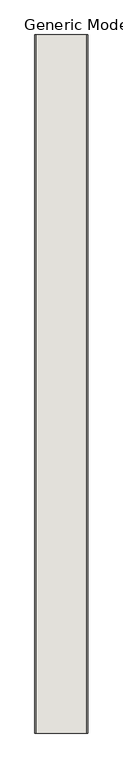
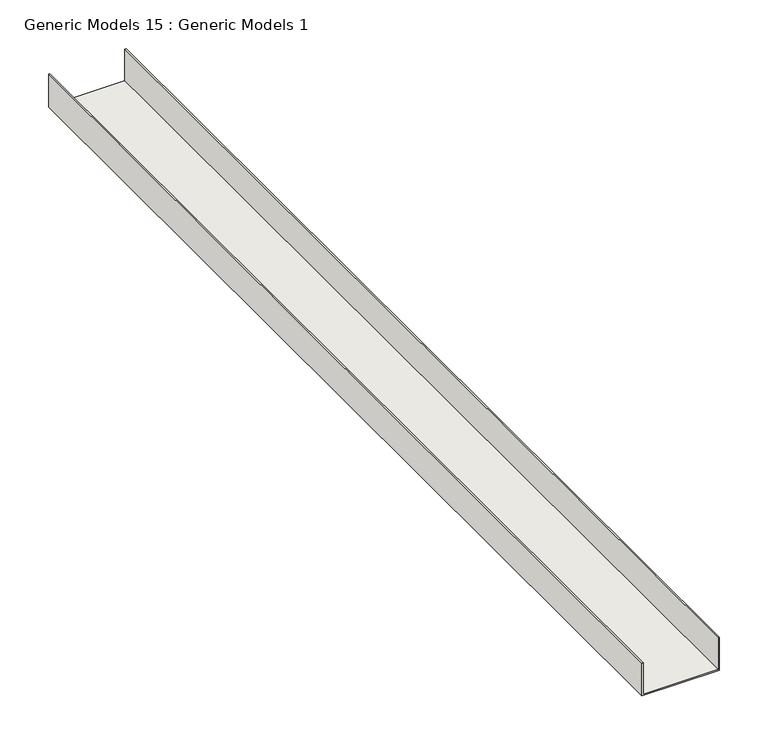
"""IFC4 building model written with IfcOpenShell, lengths in millimetres: wall geometry, Generic Models 15 : Generic Models 1."""

from ifc_helpers import new_model, si_unit, frame, origin, place, context, project, spatial, polyline, outline, extrude, source, transform, mapped, element, save


def generic_models_15_generic_models_1_38d4618c(model_context):
    return source(origin(), model_context, "Body", "SweptSolid", [
        extrude(outline(polyline([(0.0, 49784.0), (41.275, 49784.0), (41.275, 49782.4125), (1.5875, 49782.4125), (1.5875, 49693.5125), (41.275, 49693.5125), (41.275, 49691.925), (0.0, 49691.925), (0.0, 49784.0)])), frame((0.0, 0.0, 0.0), z_axis=(0.0, 1.0, 0.0), x_axis=(0.0, 0.0, 1.0)), (0.0, 0.0, 1.0), 1219.2),
    ])


if __name__ == "__main__":
    model = new_model("IFC4")
    model_context = context("Model", 3, world=origin())
    ifc_project = project(units=[si_unit("LENGTHUNIT", "METRE", prefix="MILLI")], contexts=[model_context])
    site = spatial("IfcSite", under=ifc_project)
    building = spatial("IfcBuilding", under=site)
    placement = place(None, origin())
    generic_models_15_generic_models_1_shape = generic_models_15_generic_models_1_38d4618c(model_context)
    element("IfcWall", 1, ObjectType="Generic Models 15 : Generic Models 1", at=placement, inside=building, context=model_context, shape_type="MappedRepresentation", body=[
        mapped(generic_models_15_generic_models_1_shape, transform((0.0, 0.0, 0.0), x_axis=(1.0, 0.0, 0.0), y_axis=(0.0, 1.0, 0.0), z_axis=(0.0, 0.0, 1.0))),
    ])
    save(model, "model.ifc")

# Revit data of these elements
# Element 1 (IfcWall, "Generic Models 15 : Generic Models 1")
#   Materials on its faces: "METAL RUNNER CHANNEL; FASTEN @ 24\" O.C."
# Materials
#   "METAL RUNNER CHANNEL; FASTEN @ 24\" O.C.": class "Unassigned", colour RGB 210 209 208, transparency 0, Keynote = "M05121300.02", Cost = 0
